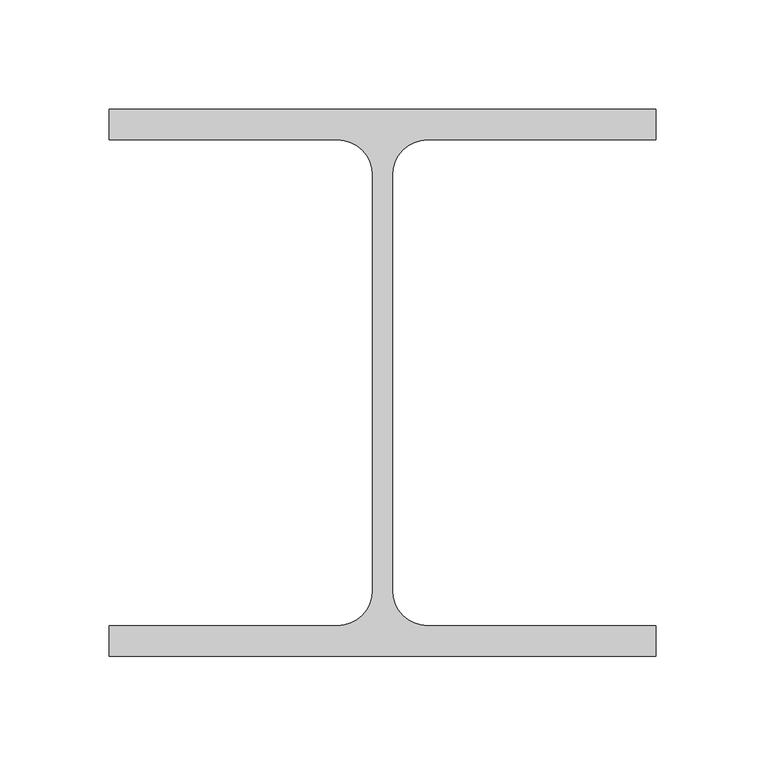
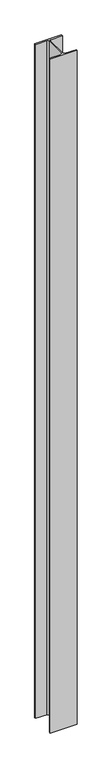
"""IFC4 building model written with IfcOpenShell, lengths in millimetres: column geometry, 0912_Steel Column_H_KSD3502 : H_SC_ASC_H-250x250x9x14."""

from ifc_helpers import new_model, si_unit, point, frame, frame_2d, origin, place, context, project, spatial, polyline, circle_curve, trimmed, segment, composite_curve, outline, extrude, source, transform, mapped, element, save


def column_8fa00422(model_context):
    return source(origin(), model_context, "Body", "SweptSolid", [
        extrude(outline(composite_curve([segment(polyline([(125.0, 125.0), (125.0, 111.0), (20.5, 111.0)]), True, "CONTINUOUS"), segment(trimmed(circle_curve(frame_2d((20.5, 95.0)), 16.0), [point((20.5, 111.0))], [point((4.5, 95.0))], True, "CARTESIAN"), True, "CONTINUOUS"), segment(polyline([(4.5, 95.0), (4.5, -95.0)]), True, "CONTINUOUS"), segment(trimmed(circle_curve(frame_2d((20.5, -95.0)), 16.0), [point((4.5, -95.0))], [point((20.5, -111.0))], True, "CARTESIAN"), True, "CONTINUOUS"), segment(polyline([(20.5, -111.0), (125.0, -111.0), (125.0, -125.0), (-125.0, -125.0), (-125.0, -111.0), (-20.5, -111.0)]), True, "CONTINUOUS"), segment(trimmed(circle_curve(frame_2d((-20.5, -95.0)), 16.0), [point((-20.5, -111.0))], [point((-4.5, -95.0))], True, "CARTESIAN"), True, "CONTINUOUS"), segment(polyline([(-4.5, -95.0), (-4.5, 95.0)]), True, "CONTINUOUS"), segment(trimmed(circle_curve(frame_2d((-20.5, 95.0)), 16.0), [point((-4.5, 95.0))], [point((-20.5, 111.0))], True, "CARTESIAN"), True, "CONTINUOUS"), segment(polyline([(-20.5, 111.0), (-125.0, 111.0), (-125.0, 125.0), (125.0, 125.0)]), True, "CONTINUOUS")], self_intersect=False)), frame((0.0, 0.0, 599.9720055), z_axis=(0.0, 0.0, 1.0), x_axis=(1.0, 0.0, 0.0)), (0.0, 0.0, 1.0), 6600.0),
    ])


if __name__ == "__main__":
    model = new_model("IFC4")
    model_context = context("Model", 3, world=origin())
    ifc_project = project(units=[si_unit("LENGTHUNIT", "METRE", prefix="MILLI")], contexts=[model_context])
    site = spatial("IfcSite", under=ifc_project)
    building = spatial("IfcBuilding", under=site)
    placement = place(None, origin())
    column_shape = column_8fa00422(model_context)
    element("IfcColumn", 1, ObjectType="0912_Steel Column_H_KSD3502 : H_SC_ASC_H-250x250x9x14", at=placement, inside=building, context=model_context, shape_type="MappedRepresentation", body=[
        mapped(column_shape, transform((0.0, 0.0, 0.0), x_axis=(1.0, 0.0, 0.0), y_axis=(0.0, 1.0, 0.0), z_axis=(0.0, 0.0, 1.0))),
    ])
    save(model, "model.ifc")

# Revit data of these elements
# Type "0912_Steel Column_H_KSD3502 : H_SC_ASC_H-250x250x9x14"
#   H_WM Code_1 = "S01AA002-00001 | Main Steel Structure Fabrication Work | Shelter/Building | Medium Steel - Standard (90KG/M>Weight≥30KG/M) | Material: (   )"
#   H_WM Code_2 = "S03AA028-00001 | Main Steel Structure Erection Work | Shelter/Building | Medium Steel (90KG/M>Weight≥30KG/M) | Material: (   )"
#   H_WM Code_3 = "S01AA010-00001 | Main Steel Structure Fabrication Work | Shelter/Building | Steel Painting/Coating | for Non-Fireproofed Steel Surface, Surface Preparation, Primer, Second & Final Coat | Material: (   )"
#   H_Q'ty Cal Type Tag = "SC-Q2"
#   Width = 25.0 cm
#   Web Thickness = 0.9 cm
#   Web Fillet = 1.6 cm
#   Warping Constant = 507646.0 cm⁶
#   Torsional Moment of Inertia = 51.4681 cm⁴
#   Section Area = 92.18 cm²
#   Plastic Modulus weak axis = 444.0 cm³
#   Plastic Modulus strong axis = 960.0 cm³
#   Perimeter = 1.46 m²/m
#   Nominal Weight = 72.40 kgf/m
#   Moment of Inertia weak axis = 3650.00 cm⁴
#   Moment of Inertia strong axis = 10800.00 cm⁴
#   Height = 25.0 cm
#   Flange Thickness = 1.4 cm
#   Elastic Modulus weak axis = 292.0 cm³
#   Elastic Modulus strong axis = 867.0 cm³
#   Centroid Vertical = 12.5 cm
#   Centroid Horizontal = 12.5 cm
#   Structural Material [instance default] = Steel, 45-345
#   Section Name Key = ""
#   Bolt Spacing = 0
#   Assembly Code = ""
# Element 1 (IfcColumn, "0912_Steel Column_H_KSD3502 : H_SC_ASC_H-250x250x9x14")
#   Structural Material = A03AD029-00005_Anchor Bolt (Installation only)_M24
#   Materials on its faces: "A03AD029-00005_Anchor Bolt (Installation only)_M24"
# Materials
#   "Steel, 45-345": class "Metal", colour RGB 189 187 185, transparency 0, Description = "Steel 345 MPa", Cost = 0
#   "A03AD029-00005_Anchor Bolt (Installation only)_M24": class "Unassigned", colour RGB 84 83 81, transparency 0, Cost = 0
